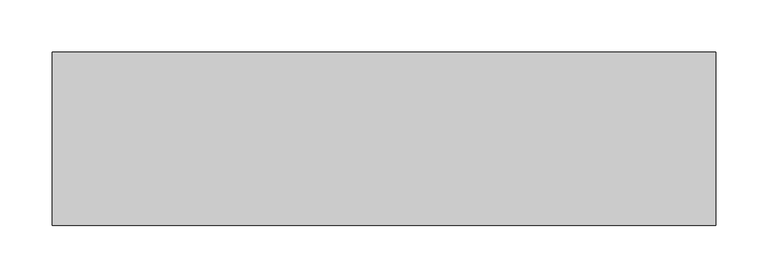
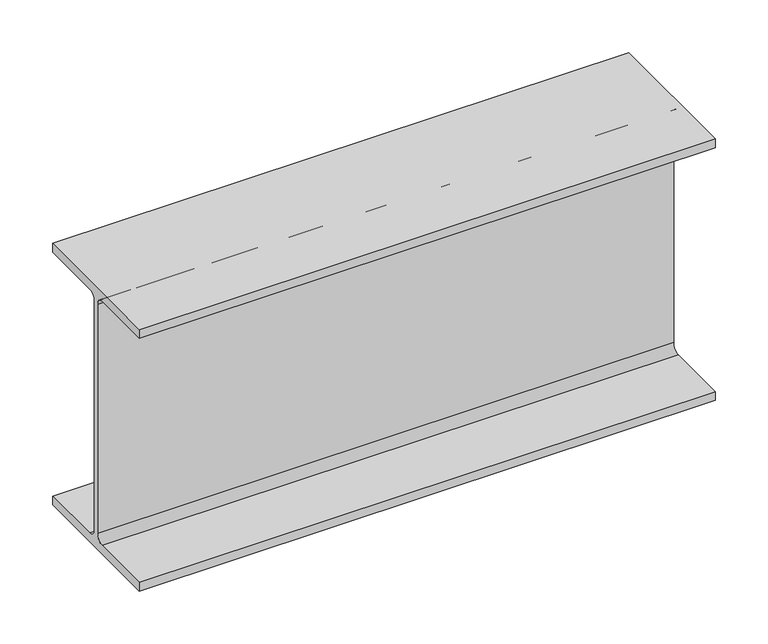
"""IFC4 building model written with IfcOpenShell, lengths in millimetres: beam geometry, Old_Steel Beam_H-KSD3502 : H_SB_ASB_H-300×150x6.5x9."""

from ifc_helpers import new_model, si_unit, point, frame, frame_2d, origin, place, context, project, spatial, polyline, circle_curve, trimmed, segment, composite_curve, outline, extrude, source, transform, mapped, element, save


def beam_fa83c41e(model_context):
    return source(origin(), model_context, "Body", "SweptSolid", [
        extrude(outline(composite_curve([segment(polyline([(82.5, -141.5), (82.5, -151.7), (-82.5, -151.7), (-82.5, -141.5), (-11.9, -141.5)]), True, "CONTINUOUS"), segment(trimmed(circle_curve(frame_2d((-11.9, -132.6)), 8.9), [point((-11.9, -141.5))], [point((-3.0, -132.6))], True, "CARTESIAN"), True, "CONTINUOUS"), segment(polyline([(-3.0, -132.6), (-3.0, 132.6)]), True, "CONTINUOUS"), segment(trimmed(circle_curve(frame_2d((-11.9, 132.6)), 8.9), [point((-3.0, 132.6))], [point((-11.9, 141.5))], True, "CARTESIAN"), True, "CONTINUOUS"), segment(polyline([(-11.9, 141.5), (-82.5, 141.5), (-82.5, 151.7), (82.5, 151.7), (82.5, 141.5), (11.9, 141.5)]), True, "CONTINUOUS"), segment(trimmed(circle_curve(frame_2d((11.9, 132.6)), 8.9), [point((11.9, 141.5))], [point((3.0, 132.6))], True, "CARTESIAN"), True, "CONTINUOUS"), segment(polyline([(3.0, 132.6), (3.0, -132.6)]), True, "CONTINUOUS"), segment(trimmed(circle_curve(frame_2d((11.9, -132.6)), 8.9), [point((3.0, -132.6))], [point((11.9, -141.5))], True, "CARTESIAN"), True, "CONTINUOUS"), segment(polyline([(11.9, -141.5), (82.5, -141.5)]), True, "CONTINUOUS")], self_intersect=False)), frame((-282.3, 0.0, 0.0), z_axis=(1.0, 0.0, 0.0), x_axis=(0.0, 1.0, 0.0)), (0.0, 0.0, 1.0), 632.1),
    ])


if __name__ == "__main__":
    model = new_model("IFC4")
    model_context = context("Model", 3, world=origin())
    ifc_project = project(units=[si_unit("LENGTHUNIT", "METRE", prefix="MILLI")], contexts=[model_context])
    site = spatial("IfcSite", under=ifc_project)
    building = spatial("IfcBuilding", under=site)
    placement = place(None, origin())
    beam_shape = beam_fa83c41e(model_context)
    element("IfcBeam", 1, ObjectType="Old_Steel Beam_H-KSD3502 : H_SB_ASB_H-300×150x6.5x9", at=placement, inside=building, context=model_context, shape_type="MappedRepresentation", body=[
        mapped(beam_shape, transform((0.0, 0.0, 0.0), x_axis=(1.0, 0.0, 0.0), y_axis=(0.0, 1.0, 0.0), z_axis=(0.0, 0.0, 1.0))),
    ])
    save(model, "model.ifc")

# Revit data of these elements
# Type "Old_Steel Beam_H-KSD3502 : H_SB_ASB_H-300×150x6.5x9"
#   Width = 15.0 cm
#   Web Thickness = 0.65 cm
#   Web Fillet = 1.3 cm
#   Warping Constant = 107174.0 cm⁶
#   Torsional Moment of Inertia = 9.9539 cm⁴
#   Torsional Modulus = 1.0 cm³
#   Section Area = 46.78 cm²
#   Plastic Modulus weak axis = 105.0 cm³
#   Plastic Modulus strong axis = 542.0 cm³
#   Perimeter = 1.17 m²/m
#   Nominal Weight = 36.70 kgf/m
#   Moment of Inertia weak axis = 508.00 cm⁴
#   Moment of Inertia strong axis = 7210.00 cm⁴
#   Height = 30.0 cm
#   Flange Thickness = 0.9 cm
#   Elastic Modulus weak axis = 67.7 cm³
#   Elastic Modulus strong axis = 481.0 cm³
#   Centroid Vertical = 15.0 cm
#   Centroid Horizontal = 7.5 cm
#   Length [instance default] = 1.5240 m
#   Structural Material [instance default] = Steel, 45-345
#   Assembly Code = ""
# Element 1 (IfcBeam, "Old_Steel Beam_H-KSD3502 : H_SB_ASB_H-300×150x6.5x9")
#   Structural Material = none
# Materials
#   "Steel, 45-345": class "Metal", colour RGB 189 187 185, transparency 0, Description = "Steel 345 MPa", Cost = 0
